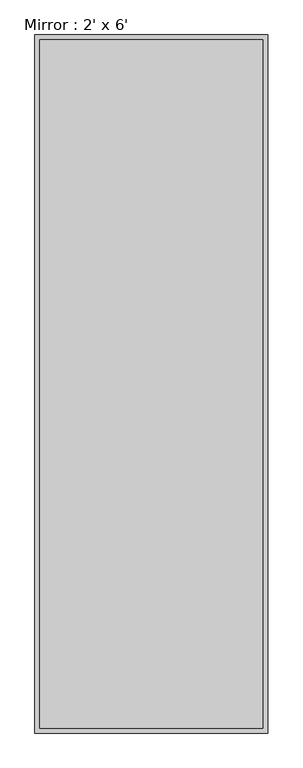
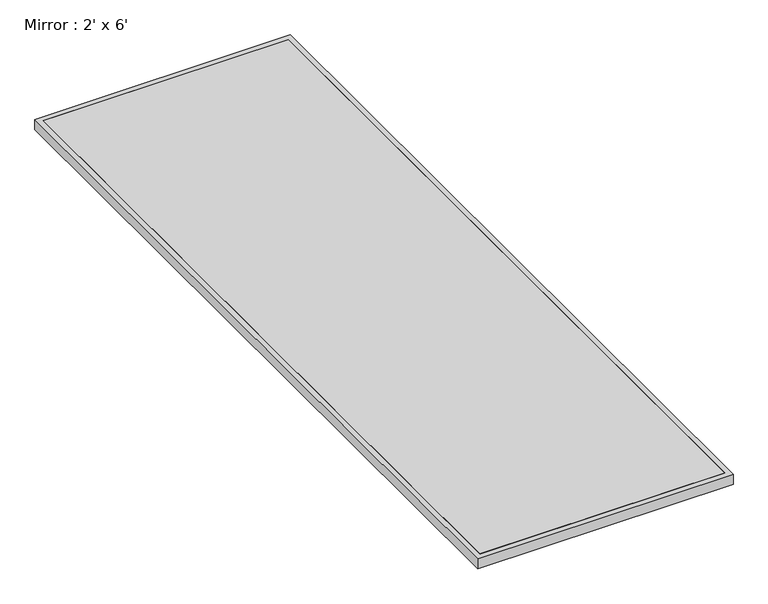
"""IFC4 building model written with IfcOpenShell, lengths in millimetres: furniture geometry, Mirror : 2' x 6'."""

from ifc_helpers import new_model, si_unit, origin, origin_with_axes, place, context, project, spatial, polyline, outline, extrude, source, transform, mapped, element, save


def mirror_2_x_6_381cc33e(model_context):
    return source(origin(), model_context, "Body", "SweptSolid", [
        extrude(outline(polyline([(292.1, -901.7), (-292.1, -901.7), (-292.1, 901.7), (292.1, 901.7), (292.1, -901.7)])), origin_with_axes(), (0.0, 0.0, 1.0), 25.4),
        extrude(outline(polyline([(304.8, -914.4), (-304.8, -914.4), (-304.8, 914.4), (304.8, 914.4), (304.8, -914.4)]), holes=[polyline([(292.1, -901.7), (292.1, 901.7), (-292.1, 901.7), (-292.1, -901.7), (292.1, -901.7)])]), origin_with_axes(), (0.0, 0.0, 1.0), 25.4),
    ])


if __name__ == "__main__":
    model = new_model("IFC4")
    model_context = context("Model", 3, world=origin())
    ifc_project = project(units=[si_unit("LENGTHUNIT", "METRE", prefix="MILLI")], contexts=[model_context])
    site = spatial("IfcSite", under=ifc_project)
    building = spatial("IfcBuilding", under=site)
    placement = place(None, origin())
    mirror_2_x_6_shape = mirror_2_x_6_381cc33e(model_context)
    element("IfcFurniture", 1, ObjectType="Mirror : 2' x 6'", at=placement, inside=building, context=model_context, shape_type="MappedRepresentation", body=[
        mapped(mirror_2_x_6_shape, transform((0.0, 0.0, 0.0), x_axis=(1.0, 0.0, 0.0), y_axis=(0.0, 1.0, 0.0), z_axis=(0.0, 0.0, 1.0))),
    ])
    save(model, "model.ifc")

# Revit data of these elements
# Type "Mirror : 2' x 6'"
#   Width = 2' - 0"
#   Height = 6' - 0"
#   Frame Thickness = 0' - 0 1/2"
#   Default Elevation = 4' - 0"
#   Mirror = Glass - Mirror
#   Frame = Metal - Chrome
# Element 1 (IfcFurniture, "Mirror : 2' x 6'")
#   Materials on its faces: "Metal - Chrome", "Glass - Mirror"
# Materials
#   "Glass - Mirror": class "Glass", colour RGB 0 128 192, transparency 0.75, Comments = "Rendering appearance not upgraded Rendering appearance not upgraded ", Description = "Glass"
#   "Metal - Chrome": class "Metal", colour RGB 244 244 244, transparency 0, Comments = "Rendering appearance not upgraded Rendering appearance not upgraded ", Description = "Chrome"
